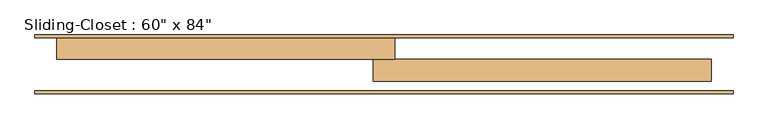
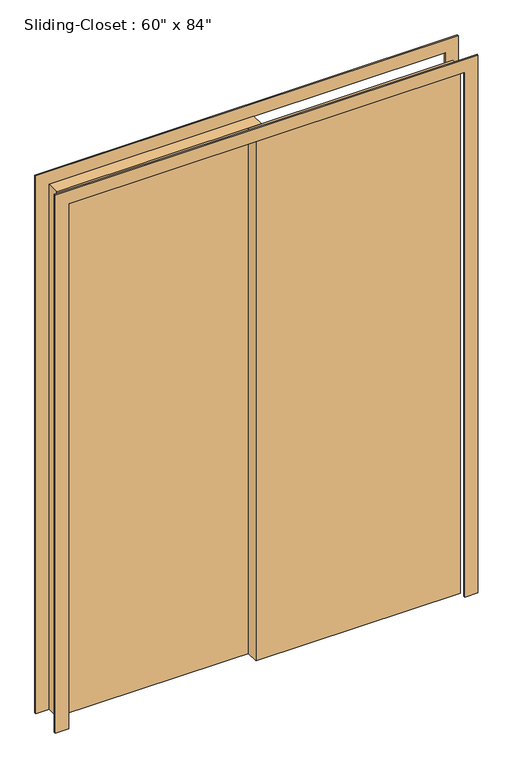
"""IFC4 building model written with IfcOpenShell, lengths in millimetres: door geometry."""

from ifc_helpers import new_model, si_unit, frame, origin, origin_with_axes, place, context, project, spatial, polyline, outline, extrude, source, transform, mapped, element, save


def door_40710fbd(model_context):
    return source(origin(), model_context, "Body", "SweptSolid", [
        extrude(outline(polyline([(-762.0, 188.9125), (25.4, 188.9125), (25.4, 138.1125), (-762.0, 138.1125), (-762.0, 188.9125)])), origin_with_axes(), (0.0, 0.0, 1.0), 2133.6),
        extrude(outline(polyline([(0.0, -812.8), (0.0, -762.0), (2133.6, -762.0), (2133.6, 762.0), (0.0, 762.0), (0.0, 812.8), (2184.4, 812.8), (2184.4, -812.8), (0.0, -812.8)])), frame((0.0, 58.7375, 0.0), z_axis=(0.0, 1.0, 0.0), x_axis=(0.0, 0.0, 1.0)), (0.0, 0.0, 1.0), 6.35),
        extrude(outline(polyline([(0.0, 812.8), (2184.4, 812.8), (2184.4, -812.8), (0.0, -812.8), (0.0, -762.0), (2133.6, -762.0), (2133.6, 762.0), (0.0, 762.0), (0.0, 812.8)])), frame((0.0, 188.9125, 0.0), z_axis=(0.0, 1.0, 0.0), x_axis=(0.0, 0.0, 1.0)), (0.0, 0.0, 1.0), 6.35),
        extrude(outline(polyline([(762.0, 87.3125), (-25.4, 87.3125), (-25.4, 138.1125), (762.0, 138.1125), (762.0, 87.3125)])), origin_with_axes(), (0.0, 0.0, 1.0), 2133.6),
    ])


if __name__ == "__main__":
    model = new_model("IFC4")
    model_context = context("Model", 3, world=origin())
    ifc_project = project(units=[si_unit("LENGTHUNIT", "METRE", prefix="MILLI")], contexts=[model_context])
    site = spatial("IfcSite", under=ifc_project)
    building = spatial("IfcBuilding", under=site)
    placement = place(None, origin())
    door_shape = door_40710fbd(model_context)
    element("IfcDoor", 1, ObjectType="Sliding-Closet : 60\" x 84\"", at=placement, inside=building, context=model_context, shape_type="MappedRepresentation", body=[
        mapped(door_shape, transform((0.0, 0.0, 0.0), x_axis=(1.0, 0.0, 0.0), y_axis=(0.0, 1.0, 0.0), z_axis=(0.0, 0.0, 1.0))),
    ])
    save(model, "model.ifc")

# Revit data of these elements
# Type "Sliding-Closet : 60\" x 84\""
#   Type Mark = "27"
#   Construction Type Id = "MDOOR"
#   Assembly Code = "C1020"
#   Analytic Construction = "Metal"
#   Thickness = 0' - 2"
#   Thermal Resistance (R) = 0.270117 (m²·K)/W
#   Heat Transfer Coefficient (U) = 3.7021 W/(m²·K)
#   Height = 7' - 0"
#   Trim Projection Ext = 0' - 0 1/4"
#   Trim Projection Int = 0' - 0 1/4"
#   Trim Width = 0' - 2"
#   Width = 5' - 0"
#   Door Material = Door - Panel
#   Frame Material = Aluminum
#   Visual Light Transmittance = 0
#   Solar Heat Gain Coefficient = 0
#   Function = (empty or 0)
#   Wall Closure = (empty or 0)
# Element 1 (IfcDoor, "Sliding-Closet : 60\" x 84\"")
#   Materials on its faces: "Aluminum", "Door - Panel"
# Materials
#   "Door - Panel": class "Wood", colour RGB 114 82 51, transparency 0
#   "Aluminum": class "Metal", colour RGB 244 244 244, transparency 0, Description = "Aluminum 6061", Cost = 0
